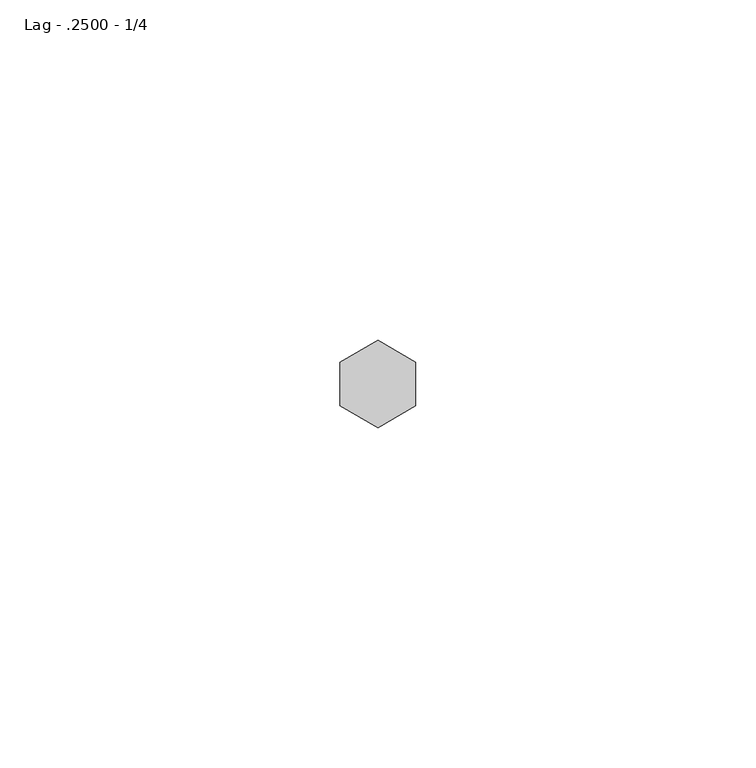
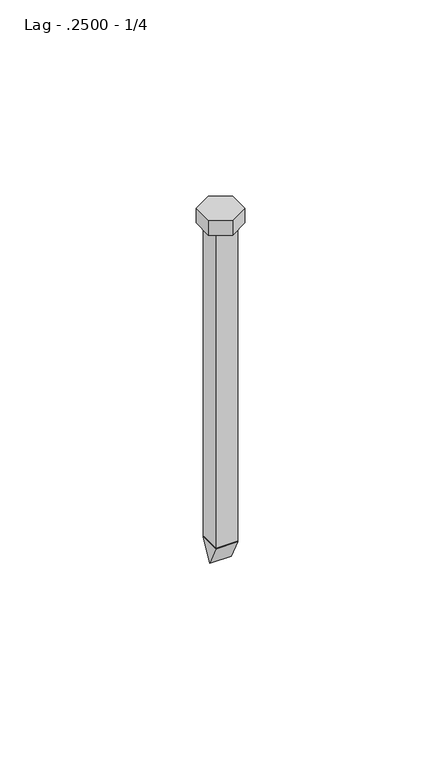
"""IFC4 building model written with IfcOpenShell, lengths in millimetres: fastener geometry, 060523 - W_P_C - Fastenings - Generic - SQUARE : Lag - .2500 - 1/4."""

from ifc_helpers import new_model, si_unit, frame, origin, origin_with_axes, place, context, project, spatial, polyline, outline, extrude, source, transform, mapped, element, save


def lag_2500_1_4_1fa157ba(model_context):
    return source(origin(), model_context, "Body", "SweptSolid", [
        extrude(outline(polyline([(0.0, -108.204), (-3.302, -101.6), (3.302, -101.6), (0.0, -108.204)])), frame((-3.302, 0.0, 0.0), z_axis=(1.0, 0.0, 0.0), x_axis=(0.0, 1.0, 0.0)), (0.0, 0.0, 1.0), 6.604),
        extrude(outline(polyline([(-5.55625, 3.2079024), (0.0, 6.4158049), (5.55625, 3.2079024), (5.55625, -3.2079024), (0.0, -6.4158049), (-5.55625, -3.2079024), (-5.55625, 3.2079024)])), origin_with_axes(), (0.0, 0.0, 1.0), 4.7625),
        extrude(outline(polyline([(-3.302, 3.302), (3.302, 3.302), (3.302, -3.302), (-3.302, -3.302), (-3.302, 3.302)])), frame((0.0, 0.0, -101.6), z_axis=(0.0, 0.0, 1.0), x_axis=(1.0, 0.0, 0.0)), (0.0, 0.0, 1.0), 101.6),
    ])


if __name__ == "__main__":
    model = new_model("IFC4")
    model_context = context("Model", 3, world=origin())
    ifc_project = project(units=[si_unit("LENGTHUNIT", "METRE", prefix="MILLI")], contexts=[model_context])
    site = spatial("IfcSite", under=ifc_project)
    building = spatial("IfcBuilding", under=site)
    placement = place(None, origin())
    lag_2500_1_4_shape = lag_2500_1_4_1fa157ba(model_context)
    element("IfcFastener", 1, ObjectType="060523 - W_P_C - Fastenings - Generic - SQUARE : Lag - .2500 - 1/4", at=placement, inside=building, context=model_context, shape_type="MappedRepresentation", body=[
        mapped(lag_2500_1_4_shape, transform((0.0, 0.0, 0.0), x_axis=(1.0, 0.0, 0.0), y_axis=(0.0, 1.0, 0.0), z_axis=(0.0, 0.0, 1.0))),
    ])
    save(model, "model.ifc")

# Revit data of these elements
# Type "060523 - W_P_C - Fastenings - Generic - SQUARE : Lag - .2500 - 1/4"
#   Washer_Thickness = 0' - 0 1/16"
#   Washer Radius = 0' - 0.3175"
#   Washer Offset - Head = 0' - 0"
#   Washer Offset = 0' - 0"
#   Thickness_of_Substrate [instance default] = 0' - 1"
#   Side = 0' - 0.25293"
#   Radius = 0' - 0.13"
#   Length [instance default] = 0' - 4"
#   Head Size = 0' - 0 7/16"
#   Head Radius = 0' - 0 7/32"
#   Head Height = 0' - 0 3/16"
#   Double Diameter = 0' - 0.52"
#   Diameter = 0' - 0.26"
#   Default Elevation = 4' - 0"
#   Washer_Nut_Visibility = no
#   Washer_Head_Visibility = no
#   Round_Head_Visibility = no
#   Point Visibility = yes
#   Nut_Visibility = no
#   Hex_Head_Visiblilty = yes
#   Washer Material = none
#   Bolt Material (Size) = AT SILL - FASTENER AT 24" O.C.
# Element 1 (IfcFastener, "060523 - W_P_C - Fastenings - Generic - SQUARE : Lag - .2500 - 1/4")
#   Materials on its faces: "AT SILL - FASTENER AT 24\" O.C."
# Materials
#   "AT SILL - FASTENER AT 24\" O.C.": class "Generic", colour RGB 120 120 120, transparency 0, Cost = 0
